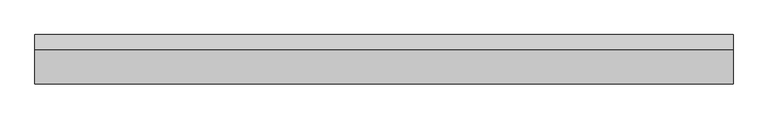
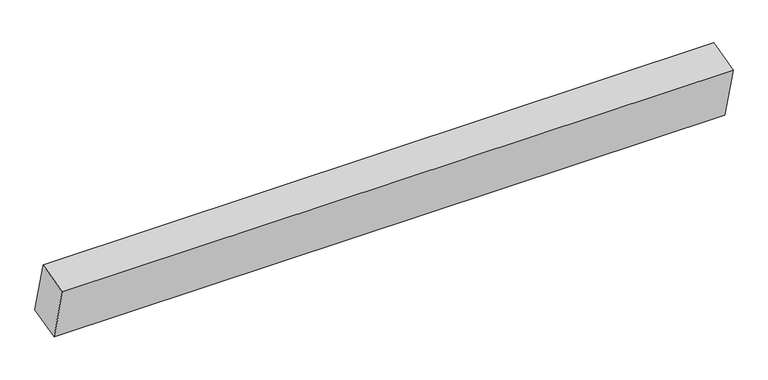
"""IFC4 building model written with IfcOpenShell, lengths in millimetres: proxy geometry, Insulation011 1113 : Insulation011 1113."""

from ifc_helpers import new_model, si_unit, frame, origin, place, context, project, spatial, polyline, outline, extrude, source, transform, mapped, element, save


def generic_models_1bf9aef2(model_context):
    return source(origin(), model_context, "Body", "SweptSolid", [
        extrude(outline(polyline([(9647.0095123, 43581.9371332), (9688.8199641, 43414.6953259), (9588.8083969, 43389.685467), (9546.9893733, 43556.9149627), (9647.0095123, 43581.9371332)])), frame((3694.2883192, 0.0, 0.0), z_axis=(1.0, 0.0, 0.0), x_axis=(0.0, 1.0, 0.0)), (0.0, 0.0, 1.0), 2000.0),
    ])


if __name__ == "__main__":
    model = new_model("IFC4")
    model_context = context("Model", 3, world=origin())
    ifc_project = project(units=[si_unit("LENGTHUNIT", "METRE", prefix="MILLI")], contexts=[model_context])
    site = spatial("IfcSite", under=ifc_project)
    building = spatial("IfcBuilding", under=site)
    placement = place(None, origin())
    generic_models_shape = generic_models_1bf9aef2(model_context)
    element("IfcBuildingElementProxy", 1, Name="Insulation011 1113 : Insulation011 1113", ObjectType="Insulation011 1113 : Insulation011 1113", at=placement, inside=building, context=model_context, shape_type="MappedRepresentation", body=[
        mapped(generic_models_shape, transform((0.0, 0.0, 0.0), x_axis=(1.0, 0.0, 0.0), y_axis=(0.0, 1.0, 0.0), z_axis=(0.0, 0.0, 1.0))),
    ])
    save(model, "model.ifc")

# Revit data of these elements
# Type "Insulation011 1113 : Insulation011 1113"
#   NameOverride = "Insulation011"
# Element 1 (IfcBuildingElementProxy, "Insulation011 1113 : Insulation011 1113")
#   Materials on its faces: "BATT INSULATION (U-FACTOR = 0.065 MIN.) OVER CLASS II VAPOR RETARDER (TOWARDS INTERIOR)"
# Materials
#   "BATT INSULATION (U-FACTOR = 0.065 MIN.) OVER CLASS II VAPOR RETARDER (TOWARDS INTERIOR)": class "Unassigned", colour RGB 246 242 160, transparency 0, Cost = 0
